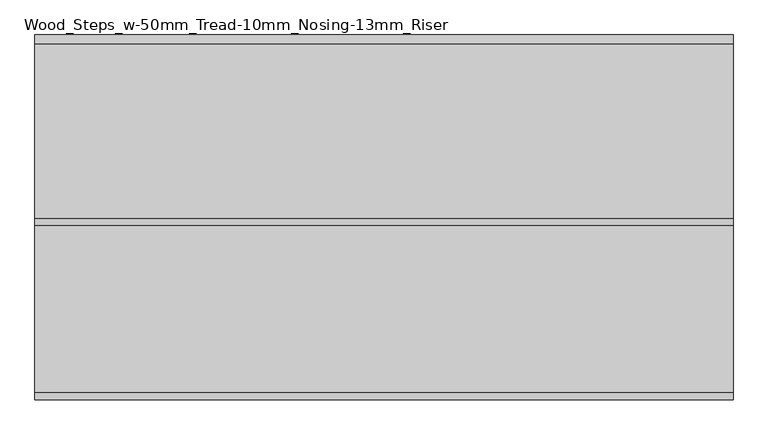
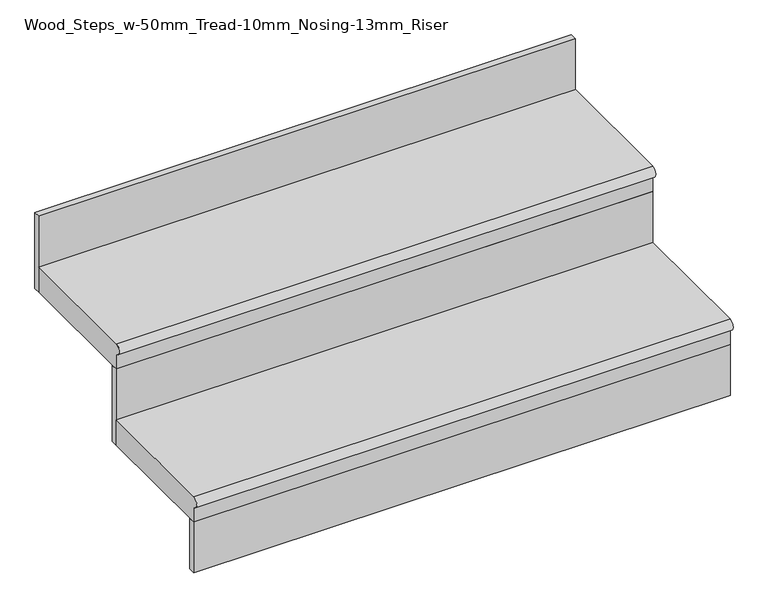
"""IFC4 building model written with IfcOpenShell, lengths in millimetres: stair flight geometry, Wood_Steps_w-50mm_Tread-10mm_Nosing-13mm_Riser."""

from ifc_helpers import new_model, si_unit, point, frame, frame_2d, origin, origin_with_axes, place, context, project, spatial, polyline, circle_curve, trimmed, segment, composite_curve, outline, extrude, source, transform, mapped, element, save


def wood_steps_w_50mm_tread_10mm_nosing_13mm_riser_c9f02b3d(model_context):
    return source(origin(), model_context, "Body", "SweptSolid", [
        extrude(outline(composite_curve([segment(polyline([(-3486.8850615, 150.0), (-3236.8850615, 150.0), (-3236.8850615, 100.0), (-3486.8850615, 100.0), (-3486.8850615, 130.0)]), True, "CONTINUOUS"), segment(trimmed(circle_curve(frame_2d((-3486.8850615, 140.0)), 10.0), [point((-3486.8850615, 130.0))], [point((-3486.8850615, 150.0))], False, "CARTESIAN"), True, "CONTINUOUS")], self_intersect=False)), frame((2002.8766391, 0.0, 0.0), z_axis=(1.0, 0.0, 0.0), x_axis=(0.0, 1.0, 0.0)), (0.0, 0.0, 1.0), 1000.0),
        extrude(outline(polyline([(3002.8766391, -3474.3850615), (3002.8766391, -3486.8850615), (2002.8766391, -3486.8850615), (2002.8766391, -3474.3850615), (3002.8766391, -3474.3850615)])), origin_with_axes(), (0.0, 0.0, 1.0), 100.0),
        extrude(outline(polyline([(3002.8766391, -3224.3850615), (3002.8766391, -3236.8850615), (2002.8766391, -3236.8850615), (2002.8766391, -3224.3850615), (3002.8766391, -3224.3850615)])), frame((0.0, 0.0, 100.0), z_axis=(0.0, 0.0, 1.0), x_axis=(1.0, 0.0, 0.0)), (0.0, 0.0, 1.0), 150.0),
        extrude(outline(polyline([(3002.8766391, -2974.3850615), (3002.8766391, -2986.8850615), (2002.8766391, -2986.8850615), (2002.8766391, -2974.3850615), (3002.8766391, -2974.3850615)])), frame((0.0, 0.0, 250.0), z_axis=(0.0, 0.0, 1.0), x_axis=(1.0, 0.0, 0.0)), (0.0, 0.0, 1.0), 150.0),
        extrude(outline(composite_curve([segment(polyline([(-3236.8850615, 300.0), (-2986.8850615, 300.0), (-2986.8850615, 250.0), (-3236.8850615, 250.0), (-3236.8850615, 280.0)]), True, "CONTINUOUS"), segment(trimmed(circle_curve(frame_2d((-3236.8850615, 290.0)), 10.0), [point((-3236.8850615, 280.0))], [point((-3236.8850615, 300.0))], False, "CARTESIAN"), True, "CONTINUOUS")], self_intersect=False)), frame((2002.8766391, 0.0, 0.0), z_axis=(1.0, 0.0, 0.0), x_axis=(0.0, 1.0, 0.0)), (0.0, 0.0, 1.0), 1000.0),
    ])


if __name__ == "__main__":
    model = new_model("IFC4")
    model_context = context("Model", 3, world=origin())
    ifc_project = project(units=[si_unit("LENGTHUNIT", "METRE", prefix="MILLI")], contexts=[model_context])
    site = spatial("IfcSite", under=ifc_project)
    building = spatial("IfcBuilding", under=site)
    placement = place(None, origin())
    wood_steps_w_50mm_tread_10mm_nosing_13mm_riser_shape = wood_steps_w_50mm_tread_10mm_nosing_13mm_riser_c9f02b3d(model_context)
    element("IfcStairFlight", 1, ObjectType="Wood_Steps_w-50mm_Tread-10mm_Nosing-13mm_Riser", at=placement, inside=building, context=model_context, shape_type="MappedRepresentation", body=[
        mapped(wood_steps_w_50mm_tread_10mm_nosing_13mm_riser_shape, transform((0.0, 0.0, 0.0), x_axis=(1.0, 0.0, 0.0), y_axis=(0.0, 1.0, 0.0), z_axis=(0.0, 0.0, 1.0))),
    ])
    save(model, "model.ifc")

# Revit data of these elements
# Element 1 (IfcStairFlight, "Wood_Steps_w-50mm_Tread-10mm_Nosing-13mm_Riser")
#   Materials on its faces: "Oak Flooring"
# Materials
#   "Oak Flooring": class "Wood", colour RGB 212 179 113, transparency 0, Description = "Quercus Rubra", Cost = 0
